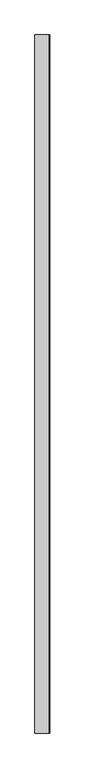
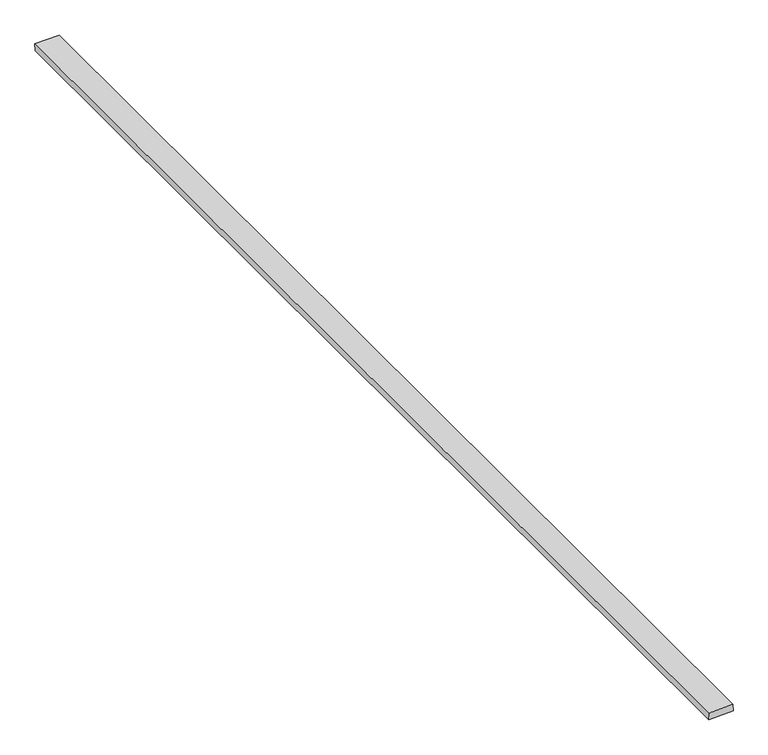
"""IFC4 building model written with IfcOpenShell, lengths in millimetres: proxy geometry, Generic Models 7:Generic Models 1:337419:Generic Models 1:337419 : Generic Models 7:Generic Models 1:337419:36 : Generic Models 7:Generic Models 1:337419:Generic Models 1:337419 : Generic Models 7:Generic Models 1:337419:301336."""

import ifcopenshell
import ifcopenshell.guid

model = None  # the IFC model being written
_history = None  # IfcOwnerHistory: only IFC2X3 demands one
_inside = {}  # id of a spatial element -> (the spatial element, [elements in it])
_under = {}  # id of a project, library or spatial element -> (it, [spatial elements below it])
_declared = {}  # id of a project -> (the project, [libraries it declares])
_typed = {}  # id of a type object -> (the type object, [elements of that type])
_made_of = {}  # id of a material, layer set ... -> (it, [elements and type objects made of it])


def new_model(schema):
    """Start an empty IFC model of exactly this schema.

    Asked for "IFC4X3", IfcOpenShell would pick the latest addendum, in which some entities
    have other attributes; the version numbers below select the first issue.
    IFC2X3 requires an IfcOwnerHistory on every rooted entity: one is made here for all.
    """
    global model, _history
    if schema == "IFC4X3":
        model = ifcopenshell.file(schema_version=(4, 3, 0, 0))
    else:
        model = ifcopenshell.file(schema=schema)
    _inside.clear()
    _under.clear()
    _declared.clear()
    _typed.clear()
    _made_of.clear()
    _history = None
    if model.schema == "IFC2X3":
        org = make("IfcOrganization", Name="unknown")
        user = make(
            "IfcPersonAndOrganization",
            ThePerson=make("IfcPerson", FamilyName="unknown"),
            TheOrganization=org,
        )
        app = make(
            "IfcApplication",
            ApplicationDeveloper=org,
            Version="unknown",
            ApplicationFullName="unknown",
            ApplicationIdentifier="unknown",
        )
        _history = make(
            "IfcOwnerHistory",
            OwningUser=user,
            OwningApplication=app,
            ChangeAction="ADDED",
            CreationDate=0,
        )
    return model


def make(cls, **values):
    """One entity of the class cls with the attributes given. An attribute that is None is left unset."""
    return model.create_entity(
        cls, **{name: value for name, value in values.items() if value is not None}
    )


def rooted(cls, **values):
    """An entity with a GlobalId (a new one), such as an element, a storey or a relation."""
    return make(cls, GlobalId=ifcopenshell.guid.new(), OwnerHistory=_history, **values)


def si_unit(unit_type, name, prefix=None):
    """IfcSIUnit, for example si_unit("LENGTHUNIT", "METRE", prefix="MILLI")."""
    return make("IfcSIUnit", UnitType=unit_type, Prefix=prefix, Name=name)


def assignment(units):
    """IfcUnitAssignment: the units of a project."""
    return None if units is None else make("IfcUnitAssignment", Units=units)


def point(xyz):
    """IfcCartesianPoint."""
    return None if xyz is None else make("IfcCartesianPoint", Coordinates=xyz)


def direction(xyz):
    """IfcDirection."""
    return None if xyz is None else make("IfcDirection", DirectionRatios=xyz)


def frame(location, z_axis=None, x_axis=None):
    """IfcAxis2Placement3D, a coordinate frame: its origin and axes. An axis left out is left unset."""
    return make(
        "IfcAxis2Placement3D",
        Location=point(location),
        Axis=direction(z_axis),
        RefDirection=direction(x_axis),
    )


def origin():
    """The frame at (0, 0, 0) with its axes left unset."""
    return frame((0.0, 0.0, 0.0))


def place(relative_to, where):
    """IfcLocalPlacement: puts the frame where relative to a parent placement (None: the world)."""
    return make(
        "IfcLocalPlacement", PlacementRelTo=relative_to, RelativePlacement=where
    )


def context(
    kind, dimensions, precision=None, world=None, true_north=None, identifier=None
):
    """IfcGeometricRepresentationContext, for example the 3D "Model" context."""
    return make(
        "IfcGeometricRepresentationContext",
        ContextIdentifier=identifier,
        ContextType=kind,
        CoordinateSpaceDimension=dimensions,
        Precision=precision,
        WorldCoordinateSystem=world,
        TrueNorth=true_north,
    )


def project(units=None, contexts=None):
    """IfcProject with its units and contexts."""
    return rooted(
        "IfcProject",
        Name="project",
        RepresentationContexts=contexts,
        UnitsInContext=assignment(units),
    )


def spatial(cls, under=None, at=None, **own):
    """A site, building, storey or space (cls), placed at a placement, below another one or the project."""
    s = rooted(cls, ObjectPlacement=at, **own)
    if under is not None:
        _under.setdefault(under.id(), (under, []))[1].append(s)
    return s


def polyline(points):
    """IfcPolyline through the points."""
    return make("IfcPolyline", Points=[point(p) for p in points])


def outline(outer, holes=None, kind="AREA"):
    """IfcArbitraryClosedProfileDef: a profile drawn as a closed curve; with holes, ...WithVoids."""
    if holes is None:
        return make("IfcArbitraryClosedProfileDef", ProfileType=kind, OuterCurve=outer)
    return make(
        "IfcArbitraryProfileDefWithVoids",
        ProfileType=kind,
        OuterCurve=outer,
        InnerCurves=holes,
    )


def extrude(swept, where, along, depth):
    """IfcExtrudedAreaSolid: the profile swept, set in the frame where, extruded along a direction by depth."""
    return make(
        "IfcExtrudedAreaSolid",
        SweptArea=swept,
        Position=where,
        ExtrudedDirection=direction(along),
        Depth=depth,
    )


def shape(context_of_items, identifier, shape_type, items):
    """IfcShapeRepresentation: the items that make up one representation, for example the "Body"."""
    return make(
        "IfcShapeRepresentation",
        ContextOfItems=context_of_items,
        RepresentationIdentifier=identifier,
        RepresentationType=shape_type,
        Items=items,
    )


def source(mapping_origin, context_of_items, identifier, shape_type, items):
    """IfcRepresentationMap: a shape defined once, which mapped items show again and again."""
    return make(
        "IfcRepresentationMap",
        MappingOrigin=mapping_origin,
        MappedRepresentation=shape(context_of_items, identifier, shape_type, items),
    )


def transform(
    local_origin,
    x_axis=None,
    y_axis=None,
    z_axis=None,
    scale=None,
    scale2=None,
    scale3=None,
    uniform=True,
):
    """IfcCartesianTransformationOperator3D, or its non-uniform kind. x_axis, y_axis, z_axis: its Axis1, 2, 3."""
    if uniform:
        return make(
            "IfcCartesianTransformationOperator3D",
            Axis1=direction(x_axis),
            Axis2=direction(y_axis),
            LocalOrigin=point(local_origin),
            Scale=scale,
            Axis3=direction(z_axis),
        )
    return make(
        "IfcCartesianTransformationOperator3DnonUniform",
        Axis1=direction(x_axis),
        Axis2=direction(y_axis),
        LocalOrigin=point(local_origin),
        Scale=scale,
        Axis3=direction(z_axis),
        Scale2=scale2,
        Scale3=scale3,
    )


def mapped(mapping_source, mapping_target):
    """IfcMappedItem: shows the shape of a source again, moved by a transform."""
    return make(
        "IfcMappedItem", MappingSource=mapping_source, MappingTarget=mapping_target
    )


def made_of(thing, what):
    """Note that an element or type object is made of a material, layer set ...; save() writes the relation."""
    if what is not None:
        _made_of.setdefault(what.id(), (what, []))[1].append(thing)
    return thing


def element(
    cls,
    number,
    at=None,
    inside=None,
    cuts=None,
    type_object=None,
    material=None,
    context=None,
    identifier="Body",
    shape_type=None,
    held_by="IfcProductDefinitionShape",
    body=None,
    shapes=None,
    **own,
):
    """One element of the class cls, such as IfcWall. Its Tag is "e" and its number.

    at: its placement. inside: the storey or other place that contains it. cuts: it is an
    opening in that element (IfcRelVoidsElement). A single representation is given by context,
    identifier, shape_type and body (its items); several are given by shapes. held_by: the class
    of the entity that holds the representations. save() writes the other relations.
    """
    e = rooted(cls, Tag="e%d" % number, ObjectPlacement=at, **own)
    if body is not None:
        shapes = [shape(context, identifier, shape_type, body)]
    if shapes is not None:
        e.Representation = make(held_by, Representations=shapes)
    if inside is not None:
        _inside.setdefault(inside.id(), (inside, []))[1].append(e)
    if cuts is not None:
        rooted(
            "IfcRelVoidsElement", RelatingBuildingElement=cuts, RelatedOpeningElement=e
        )
    if type_object is not None:
        _typed.setdefault(type_object.id(), (type_object, []))[1].append(e)
    return made_of(e, material)


def aggregate(whole, parts):
    """IfcRelAggregates: a whole, such as a stair, and the parts it consists of."""
    return rooted("IfcRelAggregates", RelatingObject=whole, RelatedObjects=parts)


def save(model, path):
    """Write the relations noted so far, then the file.

    IfcRelAggregates (storeys below a building ...), IfcRelContainedInSpatialStructure (elements
    in a storey), IfcRelDefinesByType, IfcRelAssociatesMaterial and IfcRelDeclares: one each for
    every whole, place, type object, material and project.
    """
    for whole, parts in _under.values():
        aggregate(whole, parts)
    for where, things in _inside.values():
        rooted(
            "IfcRelContainedInSpatialStructure",
            RelatedElements=things,
            RelatingStructure=where,
        )
    for kind, things in _typed.values():
        rooted("IfcRelDefinesByType", RelatedObjects=things, RelatingType=kind)
    for what, things in _made_of.values():
        rooted("IfcRelAssociatesMaterial", RelatedObjects=things, RelatingMaterial=what)
    for by, libraries in _declared.values():
        rooted("IfcRelDeclares", RelatingContext=by, RelatedDefinitions=libraries)
    model.write(path)


def generic_models_fee346f6(model_context):
    return source(origin(), model_context, "Body", "SweptSolid", [
        extrude(outline(polyline([(0.0, -85.5699146), (0.0, 0.0), (4112.7238411, 0.0), (4112.7238411, -85.5699146), (0.0, -85.5699146)])), frame((570920.1289672, -574702.7289236, 4325.4403018), z_axis=(-0.04163054471218554, 0.0, 0.9991330730923518), x_axis=(0.0, -1.0, 0.0)), (0.0, 0.0, 1.0), 25.4),
    ])


if __name__ == "__main__":
    model = new_model("IFC4")
    model_context = context("Model", 3, world=origin())
    ifc_project = project(units=[si_unit("LENGTHUNIT", "METRE", prefix="MILLI")], contexts=[model_context])
    site = spatial("IfcSite", under=ifc_project)
    building = spatial("IfcBuilding", under=site)
    placement = place(None, origin())
    generic_models_shape = generic_models_fee346f6(model_context)
    element("IfcBuildingElementProxy", 1, Name="Generic Models 7:Generic Models 1:337419:Generic Models 1:337419 : Generic Models 7:Generic Models 1:337419:36 : Generic Models 7:Generic Models 1:337419:Generic Models 1:337419 : Generic Models 7:Generic Models 1:337419:301336", ObjectType="Generic Models 7:Generic Models 1:337419:Generic Models 1:337419 : Generic Models 7:Generic Models 1:337419:36 : Generic Models 7:Generic Models 1:337419:Generic Models 1:337419 : Generic Models 7:Generic Models 1:337419:301336", at=placement, inside=building, context=model_context, shape_type="MappedRepresentation", body=[
        mapped(generic_models_shape, transform((0.0, 0.0, 0.0), x_axis=(1.0, 0.0, 0.0), y_axis=(0.0, 1.0, 0.0), z_axis=(0.0, 0.0, 1.0))),
    ])
    save(model, "model.ifc")

# Revit data of these elements
# Type "Generic Models 7:Generic Models 1:337419:Generic Models 1:337419 : Generic Models 7:Generic Models 1:337419:36 : Generic Models 7:Generic Models 1:337419:Generic Models 1:337419 : Generic Models 7:Generic Models 1:337419:301336"
#   NameOverride = "Generic Models 7:Generic Models 1:337419:Generic Models 1:337419 : Generic Models 7:Generic Models 1:337419:301336"
#   ObjectTypeOverride = "Generic Models 1:337419 : Generic Models 7:Generic Models 1:337419"
#   Reference = "Generic Models 1"
#   Tag = "301336"
# Element 1 (IfcBuildingElementProxy, "Generic Models 7:Generic Models 1:337419:Generic Models 1:337419 : Generic Models 7:Generic Models 1:337419:36 : Generic Models 7:Generic Models 1:337419:Generic Models 1:337419 : Generic Models 7:Generic Models 1:337419:301336")
#   Materials on its faces: "1\" THERMAL SPACER @ PURLIN"
# Materials
#   "1\" THERMAL SPACER @ PURLIN": class "Unassigned", colour RGB 205 188 106, transparency 0, Cost = 0
